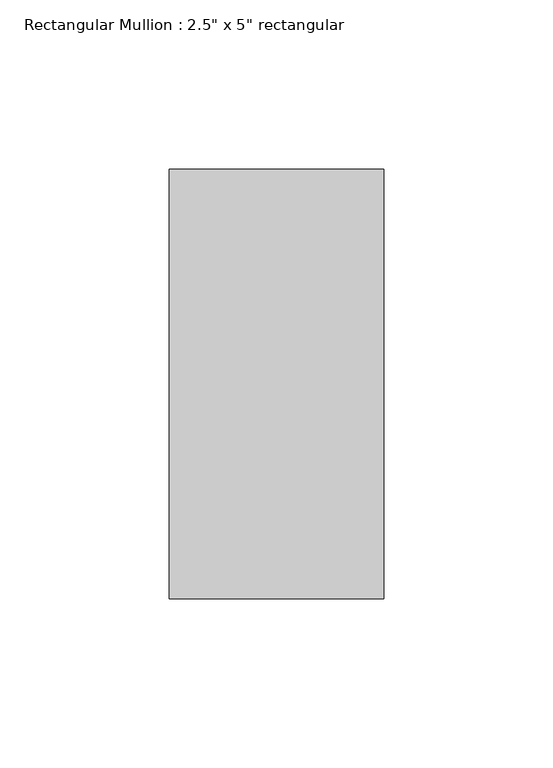
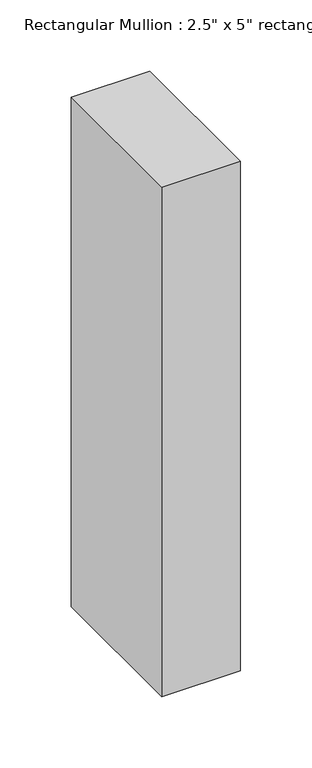
"""IFC4 building model written with IfcOpenShell, lengths in millimetres: member geometry."""

from ifc_helpers import new_model, si_unit, frame, origin, place, context, project, spatial, polyline, outline, extrude, source, transform, mapped, element, save


def member_64c4d304(model_context):
    return source(origin(), model_context, "Body", "SweptSolid", [
        extrude(outline(polyline([(0.0, 63.5), (0.0, -63.5), (-63.5, -63.5), (-63.5, 63.5), (0.0, 63.5)])), frame((0.0, 0.0, -435.6780939), z_axis=(0.0, 0.0, 1.0), x_axis=(1.0, 0.0, 0.0)), (0.0, 0.0, 1.0), 435.6780939),
    ])


if __name__ == "__main__":
    model = new_model("IFC4")
    model_context = context("Model", 3, world=origin())
    ifc_project = project(units=[si_unit("LENGTHUNIT", "METRE", prefix="MILLI")], contexts=[model_context])
    site = spatial("IfcSite", under=ifc_project)
    building = spatial("IfcBuilding", under=site)
    placement = place(None, origin())
    member_shape = member_64c4d304(model_context)
    element("IfcMember", 1, ObjectType="Rectangular Mullion : 2.5\" x 5\" rectangular", at=placement, inside=building, context=model_context, shape_type="MappedRepresentation", body=[
        mapped(member_shape, transform((0.0, 0.0, 0.0), x_axis=(1.0, 0.0, 0.0), y_axis=(0.0, 1.0, 0.0), z_axis=(0.0, 0.0, 1.0))),
    ])
    save(model, "model.ifc")

# Revit data of these elements
# Type "Rectangular Mullion : 2.5\" x 5\" rectangular"
#   built-in parameter 1007304 = 0.416667 (stored number, unit not read)
#   built-in parameter 1007301 = 0.104167 (stored number, unit not read)
#   built-in parameter 1007300 = 0.104167 (stored number, unit not read)
# Element 1 (IfcMember, "Rectangular Mullion : 2.5\" x 5\" rectangular")
#   Materials on its faces: "Metal - Aluminum 2"
# Materials
#   "Metal - Aluminum 2": class "Metal", colour RGB 189 187 185, transparency 0
